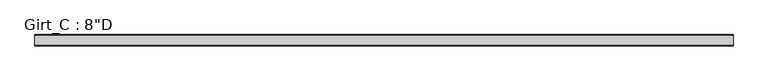
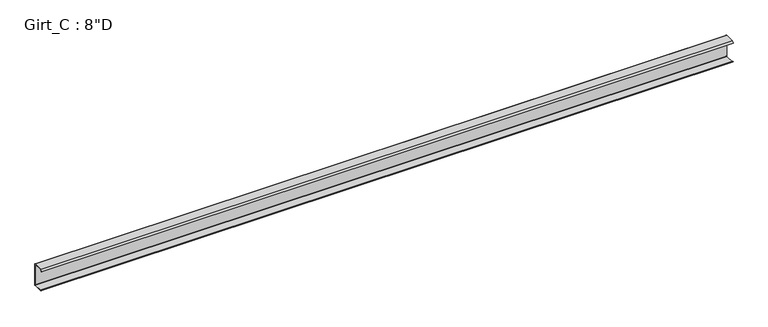
"""IFC4 building model written with IfcOpenShell, lengths in millimetres: beam geometry."""

import ifcopenshell
import ifcopenshell.guid

model = None  # the IFC model being written
_history = None  # IfcOwnerHistory: only IFC2X3 demands one
_inside = {}  # id of a spatial element -> (the spatial element, [elements in it])
_under = {}  # id of a project, library or spatial element -> (it, [spatial elements below it])
_declared = {}  # id of a project -> (the project, [libraries it declares])
_typed = {}  # id of a type object -> (the type object, [elements of that type])
_made_of = {}  # id of a material, layer set ... -> (it, [elements and type objects made of it])


def new_model(schema):
    """Start an empty IFC model of exactly this schema.

    Asked for "IFC4X3", IfcOpenShell would pick the latest addendum, in which some entities
    have other attributes; the version numbers below select the first issue.
    IFC2X3 requires an IfcOwnerHistory on every rooted entity: one is made here for all.
    """
    global model, _history
    if schema == "IFC4X3":
        model = ifcopenshell.file(schema_version=(4, 3, 0, 0))
    else:
        model = ifcopenshell.file(schema=schema)
    _inside.clear()
    _under.clear()
    _declared.clear()
    _typed.clear()
    _made_of.clear()
    _history = None
    if model.schema == "IFC2X3":
        org = make("IfcOrganization", Name="unknown")
        user = make(
            "IfcPersonAndOrganization",
            ThePerson=make("IfcPerson", FamilyName="unknown"),
            TheOrganization=org,
        )
        app = make(
            "IfcApplication",
            ApplicationDeveloper=org,
            Version="unknown",
            ApplicationFullName="unknown",
            ApplicationIdentifier="unknown",
        )
        _history = make(
            "IfcOwnerHistory",
            OwningUser=user,
            OwningApplication=app,
            ChangeAction="ADDED",
            CreationDate=0,
        )
    return model


def make(cls, **values):
    """One entity of the class cls with the attributes given. An attribute that is None is left unset."""
    return model.create_entity(
        cls, **{name: value for name, value in values.items() if value is not None}
    )


def rooted(cls, **values):
    """An entity with a GlobalId (a new one), such as an element, a storey or a relation."""
    return make(cls, GlobalId=ifcopenshell.guid.new(), OwnerHistory=_history, **values)


def si_unit(unit_type, name, prefix=None):
    """IfcSIUnit, for example si_unit("LENGTHUNIT", "METRE", prefix="MILLI")."""
    return make("IfcSIUnit", UnitType=unit_type, Prefix=prefix, Name=name)


def assignment(units):
    """IfcUnitAssignment: the units of a project."""
    return None if units is None else make("IfcUnitAssignment", Units=units)


def point(xyz):
    """IfcCartesianPoint."""
    return None if xyz is None else make("IfcCartesianPoint", Coordinates=xyz)


def direction(xyz):
    """IfcDirection."""
    return None if xyz is None else make("IfcDirection", DirectionRatios=xyz)


def frame(location, z_axis=None, x_axis=None):
    """IfcAxis2Placement3D, a coordinate frame: its origin and axes. An axis left out is left unset."""
    return make(
        "IfcAxis2Placement3D",
        Location=point(location),
        Axis=direction(z_axis),
        RefDirection=direction(x_axis),
    )


def frame_2d(location, x_axis=None):
    """IfcAxis2Placement2D, a coordinate frame in the plane: its origin and x axis."""
    return make(
        "IfcAxis2Placement2D", Location=point(location), RefDirection=direction(x_axis)
    )


def origin():
    """The frame at (0, 0, 0) with its axes left unset."""
    return frame((0.0, 0.0, 0.0))


def place(relative_to, where):
    """IfcLocalPlacement: puts the frame where relative to a parent placement (None: the world)."""
    return make(
        "IfcLocalPlacement", PlacementRelTo=relative_to, RelativePlacement=where
    )


def context(
    kind, dimensions, precision=None, world=None, true_north=None, identifier=None
):
    """IfcGeometricRepresentationContext, for example the 3D "Model" context."""
    return make(
        "IfcGeometricRepresentationContext",
        ContextIdentifier=identifier,
        ContextType=kind,
        CoordinateSpaceDimension=dimensions,
        Precision=precision,
        WorldCoordinateSystem=world,
        TrueNorth=true_north,
    )


def project(units=None, contexts=None):
    """IfcProject with its units and contexts."""
    return rooted(
        "IfcProject",
        Name="project",
        RepresentationContexts=contexts,
        UnitsInContext=assignment(units),
    )


def spatial(cls, under=None, at=None, **own):
    """A site, building, storey or space (cls), placed at a placement, below another one or the project."""
    s = rooted(cls, ObjectPlacement=at, **own)
    if under is not None:
        _under.setdefault(under.id(), (under, []))[1].append(s)
    return s


def polyline(points):
    """IfcPolyline through the points."""
    return make("IfcPolyline", Points=[point(p) for p in points])


def circle_curve(where, radius):
    """IfcCircle in the frame where."""
    return make("IfcCircle", Position=where, Radius=radius)


def trimmed(basis, trim1, trim2, sense, master):
    """IfcTrimmedCurve: the piece of a basis curve between two trims."""
    return make(
        "IfcTrimmedCurve",
        BasisCurve=basis,
        Trim1=trim1,
        Trim2=trim2,
        SenseAgreement=sense,
        MasterRepresentation=master,
    )


def segment(curve, same_sense, transition):
    """IfcCompositeCurveSegment."""
    return make(
        "IfcCompositeCurveSegment",
        Transition=transition,
        SameSense=same_sense,
        ParentCurve=curve,
    )


def composite_curve(segments, self_intersect=None):
    """IfcCompositeCurve: segments joined end to end."""
    return make("IfcCompositeCurve", Segments=segments, SelfIntersect=self_intersect)


def outline(outer, holes=None, kind="AREA"):
    """IfcArbitraryClosedProfileDef: a profile drawn as a closed curve; with holes, ...WithVoids."""
    if holes is None:
        return make("IfcArbitraryClosedProfileDef", ProfileType=kind, OuterCurve=outer)
    return make(
        "IfcArbitraryProfileDefWithVoids",
        ProfileType=kind,
        OuterCurve=outer,
        InnerCurves=holes,
    )


def extrude(swept, where, along, depth):
    """IfcExtrudedAreaSolid: the profile swept, set in the frame where, extruded along a direction by depth."""
    return make(
        "IfcExtrudedAreaSolid",
        SweptArea=swept,
        Position=where,
        ExtrudedDirection=direction(along),
        Depth=depth,
    )


def shape(context_of_items, identifier, shape_type, items):
    """IfcShapeRepresentation: the items that make up one representation, for example the "Body"."""
    return make(
        "IfcShapeRepresentation",
        ContextOfItems=context_of_items,
        RepresentationIdentifier=identifier,
        RepresentationType=shape_type,
        Items=items,
    )


def source(mapping_origin, context_of_items, identifier, shape_type, items):
    """IfcRepresentationMap: a shape defined once, which mapped items show again and again."""
    return make(
        "IfcRepresentationMap",
        MappingOrigin=mapping_origin,
        MappedRepresentation=shape(context_of_items, identifier, shape_type, items),
    )


def transform(
    local_origin,
    x_axis=None,
    y_axis=None,
    z_axis=None,
    scale=None,
    scale2=None,
    scale3=None,
    uniform=True,
):
    """IfcCartesianTransformationOperator3D, or its non-uniform kind. x_axis, y_axis, z_axis: its Axis1, 2, 3."""
    if uniform:
        return make(
            "IfcCartesianTransformationOperator3D",
            Axis1=direction(x_axis),
            Axis2=direction(y_axis),
            LocalOrigin=point(local_origin),
            Scale=scale,
            Axis3=direction(z_axis),
        )
    return make(
        "IfcCartesianTransformationOperator3DnonUniform",
        Axis1=direction(x_axis),
        Axis2=direction(y_axis),
        LocalOrigin=point(local_origin),
        Scale=scale,
        Axis3=direction(z_axis),
        Scale2=scale2,
        Scale3=scale3,
    )


def mapped(mapping_source, mapping_target):
    """IfcMappedItem: shows the shape of a source again, moved by a transform."""
    return make(
        "IfcMappedItem", MappingSource=mapping_source, MappingTarget=mapping_target
    )


def made_of(thing, what):
    """Note that an element or type object is made of a material, layer set ...; save() writes the relation."""
    if what is not None:
        _made_of.setdefault(what.id(), (what, []))[1].append(thing)
    return thing


def element(
    cls,
    number,
    at=None,
    inside=None,
    cuts=None,
    type_object=None,
    material=None,
    context=None,
    identifier="Body",
    shape_type=None,
    held_by="IfcProductDefinitionShape",
    body=None,
    shapes=None,
    **own,
):
    """One element of the class cls, such as IfcWall. Its Tag is "e" and its number.

    at: its placement. inside: the storey or other place that contains it. cuts: it is an
    opening in that element (IfcRelVoidsElement). A single representation is given by context,
    identifier, shape_type and body (its items); several are given by shapes. held_by: the class
    of the entity that holds the representations. save() writes the other relations.
    """
    e = rooted(cls, Tag="e%d" % number, ObjectPlacement=at, **own)
    if body is not None:
        shapes = [shape(context, identifier, shape_type, body)]
    if shapes is not None:
        e.Representation = make(held_by, Representations=shapes)
    if inside is not None:
        _inside.setdefault(inside.id(), (inside, []))[1].append(e)
    if cuts is not None:
        rooted(
            "IfcRelVoidsElement", RelatingBuildingElement=cuts, RelatedOpeningElement=e
        )
    if type_object is not None:
        _typed.setdefault(type_object.id(), (type_object, []))[1].append(e)
    return made_of(e, material)


def aggregate(whole, parts):
    """IfcRelAggregates: a whole, such as a stair, and the parts it consists of."""
    return rooted("IfcRelAggregates", RelatingObject=whole, RelatedObjects=parts)


def save(model, path):
    """Write the relations noted so far, then the file.

    IfcRelAggregates (storeys below a building ...), IfcRelContainedInSpatialStructure (elements
    in a storey), IfcRelDefinesByType, IfcRelAssociatesMaterial and IfcRelDeclares: one each for
    every whole, place, type object, material and project.
    """
    for whole, parts in _under.values():
        aggregate(whole, parts)
    for where, things in _inside.values():
        rooted(
            "IfcRelContainedInSpatialStructure",
            RelatedElements=things,
            RelatingStructure=where,
        )
    for kind, things in _typed.values():
        rooted("IfcRelDefinesByType", RelatedObjects=things, RelatingType=kind)
    for what, things in _made_of.values():
        rooted("IfcRelAssociatesMaterial", RelatedObjects=things, RelatingMaterial=what)
    for by, libraries in _declared.values():
        rooted("IfcRelDeclares", RelatingContext=by, RelatedDefinitions=libraries)
    model.write(path)


def beam_169d596a(model_context):
    return source(origin(), model_context, "Body", "SweptSolid", [
        extrude(outline(composite_curve([segment(polyline([(-87.5109375, 101.6), (-3.3734375, 101.6)]), True, "CONTINUOUS"), segment(trimmed(circle_curve(frame_2d((-3.3734375, 96.8375)), 4.7625), [point((-3.3734375, 101.6))], [point((1.3890625, 96.8375))], False, "CARTESIAN"), True, "CONTINUOUS"), segment(polyline([(1.3890625, 96.8375), (1.3890625, -96.8375)]), True, "CONTINUOUS"), segment(trimmed(circle_curve(frame_2d((-3.3734375, -96.8375)), 4.7625), [point((1.3890625, -96.8375))], [point((-3.3734375, -101.6))], False, "CARTESIAN"), True, "CONTINUOUS"), segment(polyline([(-3.3734375, -101.6), (-87.5109375, -101.6), (-99.7792647, -86.979177), (-97.6510975, -85.1934327), (-86.2154765, -98.821875), (-3.2694106, -98.821875)]), True, "CONTINUOUS"), segment(trimmed(circle_curve(frame_2d((-3.3748024, -96.8389339)), 1.9857399), [point((-3.2694106, -98.821875))], [point((-1.3890625, -96.8389339))], True, "CARTESIAN"), True, "CONTINUOUS"), segment(polyline([(-1.3890625, -96.8389339), (-1.3890625, 96.8381931)]), True, "CONTINUOUS"), segment(trimmed(circle_curve(frame_2d((-3.3741066, 96.8381931)), 1.9850441), [point((-1.3890625, 96.8381931))], [point((-3.3005807, 98.821875))], True, "CARTESIAN"), True, "CONTINUOUS"), segment(polyline([(-3.3005807, 98.821875), (-86.2154765, 98.821875), (-97.6278742, 85.221109), (-99.7560415, 87.0068534), (-87.5109375, 101.6)]), True, "CONTINUOUS")], self_intersect=False)), frame((-3100.3875, 0.0, 0.0), z_axis=(1.0, 0.0, 0.0), x_axis=(0.0, 1.0, 0.0)), (0.0, 0.0, 1.0), 6128.639),
    ])


if __name__ == "__main__":
    model = new_model("IFC4")
    model_context = context("Model", 3, world=origin())
    ifc_project = project(units=[si_unit("LENGTHUNIT", "METRE", prefix="MILLI")], contexts=[model_context])
    site = spatial("IfcSite", under=ifc_project)
    building = spatial("IfcBuilding", under=site)
    placement = place(None, origin())
    beam_shape = beam_169d596a(model_context)
    element("IfcBeam", 1, ObjectType="Girt_C : 8\"D", at=placement, inside=building, context=model_context, shape_type="MappedRepresentation", body=[
        mapped(beam_shape, transform((0.0, 0.0, 0.0), x_axis=(1.0, 0.0, 0.0), y_axis=(0.0, 1.0, 0.0), z_axis=(0.0, 0.0, 1.0))),
    ])
    save(model, "model.ifc")

# Revit data of these elements
# Type "Girt_C : 8\"D"
#   half leg = 0' - 1 3/4"
#   Web_Thickness = 0' - 0 7/64"
#   Length [instance default] = 10' - 0"
#   Leg_1 = 0' - 3 1/2"
#   Height = 0' - 8"
#   Structural Material [instance default] = none
# Element 1 (IfcBeam, "Girt_C : 8\"D")
#   Structural Material = CEE' SECTION (8.0x3.5C - SEE STRUCT. DWGS)
#   Materials on its faces: "CEE' SECTION (8.0x3.5C - SEE STRUCT. DWGS)"
# Materials
#   "CEE' SECTION (8.0x3.5C - SEE STRUCT. DWGS)": class "Metal", colour RGB 137 146 153, transparency 0, Description = "Steel, mill finish", Cost = 0
